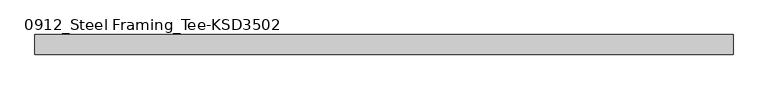
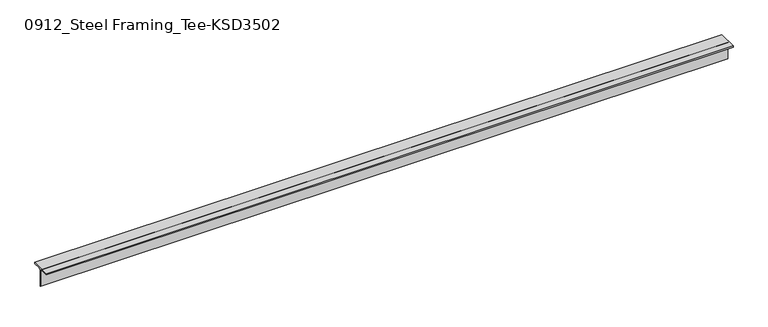
"""IFC4 building model written with IfcOpenShell, lengths in millimetres: member geometry, 0912_Steel Framing_Tee-KSD3502 : H_SB_ASB_CT-150x150x6.5x9."""

from ifc_helpers import new_model, si_unit, point, frame, frame_2d, origin, place, context, project, spatial, polyline, circle_curve, trimmed, segment, composite_curve, outline, extrude, source, transform, mapped, element, save


def member_0912_steel_framing_tee_ksd3502_bebd5093(model_context):
    return source(origin(), model_context, "Body", "SweptSolid", [
        extrude(outline(composite_curve([segment(polyline([(-75.0, 75.0), (75.0, 75.0), (75.0, 66.0), (16.25, 66.0)]), True, "CONTINUOUS"), segment(trimmed(circle_curve(frame_2d((16.25, 53.0)), 13.0), [point((16.25, 66.0))], [point((3.25, 53.0))], True, "CARTESIAN"), True, "CONTINUOUS"), segment(polyline([(3.25, 53.0), (3.25, -75.0), (-3.25, -75.0), (-3.25, 53.0)]), True, "CONTINUOUS"), segment(trimmed(circle_curve(frame_2d((-16.25, 53.0)), 13.0), [point((-3.25, 53.0))], [point((-16.25, 66.0))], True, "CARTESIAN"), True, "CONTINUOUS"), segment(polyline([(-16.25, 66.0), (-75.0, 66.0), (-75.0, 75.0)]), True, "CONTINUOUS")], self_intersect=False)), frame((-2743.0, 0.0, 0.0), z_axis=(1.0, 0.0, 0.0), x_axis=(0.0, 1.0, 0.0)), (0.0, 0.0, 1.0), 5331.5),
    ])


if __name__ == "__main__":
    model = new_model("IFC4")
    model_context = context("Model", 3, world=origin())
    ifc_project = project(units=[si_unit("LENGTHUNIT", "METRE", prefix="MILLI")], contexts=[model_context])
    site = spatial("IfcSite", under=ifc_project)
    building = spatial("IfcBuilding", under=site)
    placement = place(None, origin())
    member_0912_steel_framing_tee_ksd3502_shape = member_0912_steel_framing_tee_ksd3502_bebd5093(model_context)
    element("IfcMember", 1, ObjectType="0912_Steel Framing_Tee-KSD3502 : H_SB_ASB_CT-150x150x6.5x9", at=placement, inside=building, context=model_context, shape_type="MappedRepresentation", body=[
        mapped(member_0912_steel_framing_tee_ksd3502_shape, transform((0.0, 0.0, 0.0), x_axis=(1.0, 0.0, 0.0), y_axis=(0.0, 1.0, 0.0), z_axis=(0.0, 0.0, 1.0))),
    ])
    save(model, "model.ifc")

# Revit data of these elements
# Type "0912_Steel Framing_Tee-KSD3502 : H_SB_ASB_CT-150x150x6.5x9"
#   H_WM Code_1 = "S01AA003-00001 | Main Steel Structure Fabrication Work | Shelter/Building | Light Steel - Standard (30KG/M>Weight) | Material: (   )"
#   H_WM Code_2 = "S03AA029-00001 | Main Steel Structure Erection Work | Shelter/Building | Light Steel (30KG/M>Weight) | Material: (   )"
#   H_WM Code_3 = "S01AA010-00001 | Main Steel Structure Fabrication Work | Shelter/Building | Steel Painting/Coating | for Non-Fireproofed Steel Surface, Surface Preparation, Primer, Second & Final Coat | Material: (   )"
#   H_Q'ty Cal Type Tag = "SB-Q2"
#   Width = 15.0 cm
#   Web Thickness = 0.65 cm
#   Web Fillet = 1.3 cm
#   Section Area = 23.39 cm²
#   Perimeter = 0.60 m²/m
#   Nominal Weight = 18.40 kgf/m
#   Height = 15.0 cm
#   Flange Thickness = 0.9 cm
#   Centroid Vertical = 7.5 cm
#   Centroid Horizontal = 7.5 cm
#   Length [instance default] = 1.5000 m
#   Structural Material [instance default] = Steel, 45-345
#   Warping Constant = (empty or 0)
#   Torsional Moment of Inertia = 0
#   Section Name Key = ""
#   Plastic Modulus weak axis = 0
#   Plastic Modulus strong axis = 0
#   Moment of Inertia weak axis = 0
#   Moment of Inertia strong axis = 0
#   Elastic Modulus weak axis = 0
#   Elastic Modulus strong axis = 0
#   Bolt Spacing = 0
#   Assembly Code = ""
# Element 1 (IfcMember, "0912_Steel Framing_Tee-KSD3502 : H_SB_ASB_CT-150x150x6.5x9")
#   Structural Material = none
# Materials
#   "Steel, 45-345": class "Metal", colour RGB 189 187 185, transparency 0, Description = "Steel 345 MPa", Cost = 0
